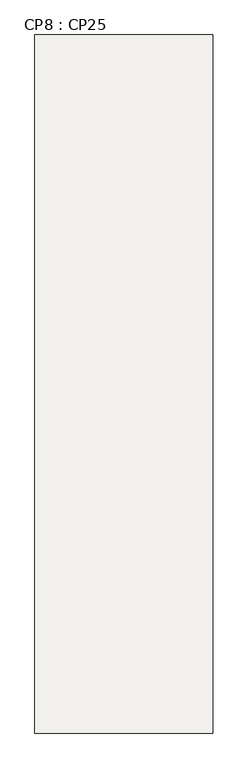
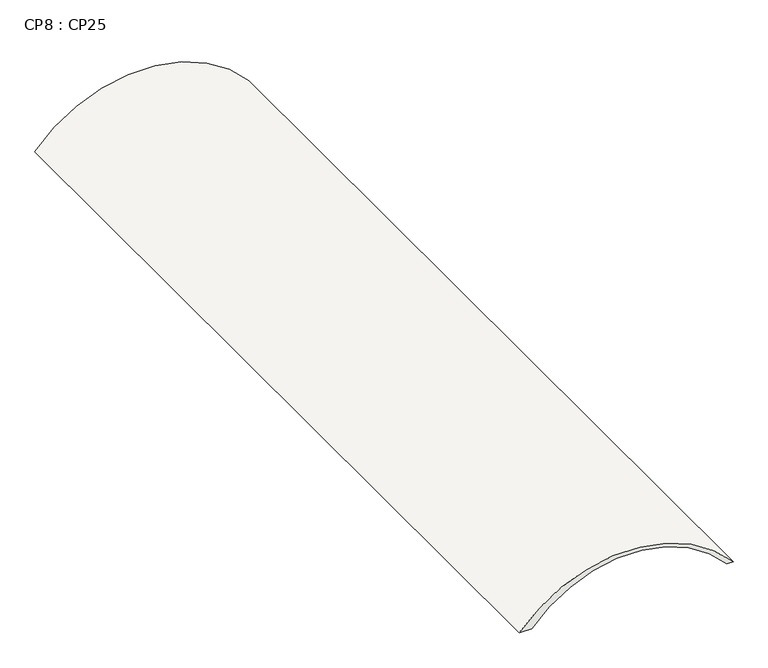
"""IFC4 building model written with IfcOpenShell, lengths in millimetres: slab geometry, CP8 : CP25."""

from ifc_helpers import new_model, si_unit, point, frame, frame_2d, origin, place, context, project, spatial, polyline, circle_curve, trimmed, segment, composite_curve, outline, extrude, source, transform, mapped, element, save


def cp8_cp25_fd1def17(model_context):
    return source(origin(), model_context, "Body", "SweptSolid", [
        extrude(outline(composite_curve([segment(polyline([(14620.0, 25183.2245516), (14620.0, 25483.2245516)]), True, "CONTINUOUS"), segment(trimmed(circle_curve(frame_2d((12608.2612414, 27833.2245515)), 3093.4758497), [point((14620.0, 25483.2245516))], [point((14620.0, 30183.2245515))], True, "CARTESIAN"), True, "CONTINUOUS"), segment(polyline([(14620.0, 30183.2245515), (14620.0, 30333.2245515)]), True, "CONTINUOUS"), segment(trimmed(circle_curve(frame_2d((12402.7966103, 27758.2245515)), 3398.0311757), [point((14620.0, 30333.2245515))], [point((14620.0, 25183.2245516))], False, "CARTESIAN"), True, "CONTINUOUS")], self_intersect=False)), frame((0.0, -100.2551788, 0.0), z_axis=(0.0, 1.0, 0.0), x_axis=(0.0, 0.0, 1.0)), (0.0, 0.0, 1.0), 20199.9999981),
    ])


if __name__ == "__main__":
    model = new_model("IFC4")
    model_context = context("Model", 3, world=origin())
    ifc_project = project(units=[si_unit("LENGTHUNIT", "METRE", prefix="MILLI")], contexts=[model_context])
    site = spatial("IfcSite", under=ifc_project)
    building = spatial("IfcBuilding", under=site)
    placement = place(None, origin())
    cp8_cp25_shape = cp8_cp25_fd1def17(model_context)
    element("IfcSlab", 1, ObjectType="CP8 : CP25", at=placement, inside=building, context=model_context, shape_type="MappedRepresentation", body=[
        mapped(cp8_cp25_shape, transform((0.0, 0.0, 0.0), x_axis=(1.0, 0.0, 0.0), y_axis=(0.0, 1.0, 0.0), z_axis=(0.0, 0.0, 1.0))),
    ])
    save(model, "model.ifc")

# Revit data of these elements
# Element 1 (IfcSlab, "CP8 : CP25")
#   Materials on its faces: "Concrete, RC"
# Materials
#   "Concrete, RC": class "Concrete", colour RGB 128 128 128, transparency 0, Description = "Cast-in-place concrete", Cost = 0
